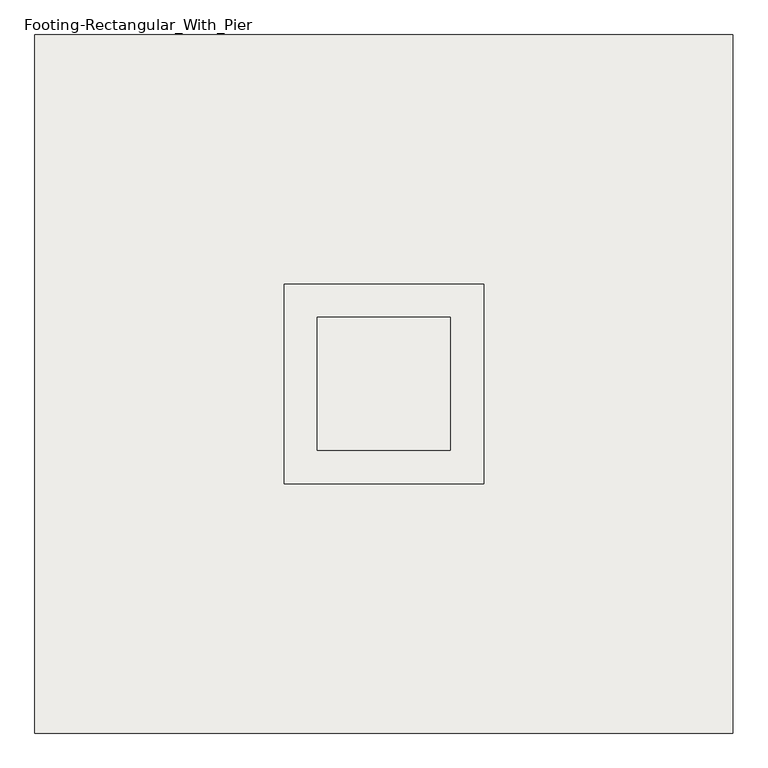
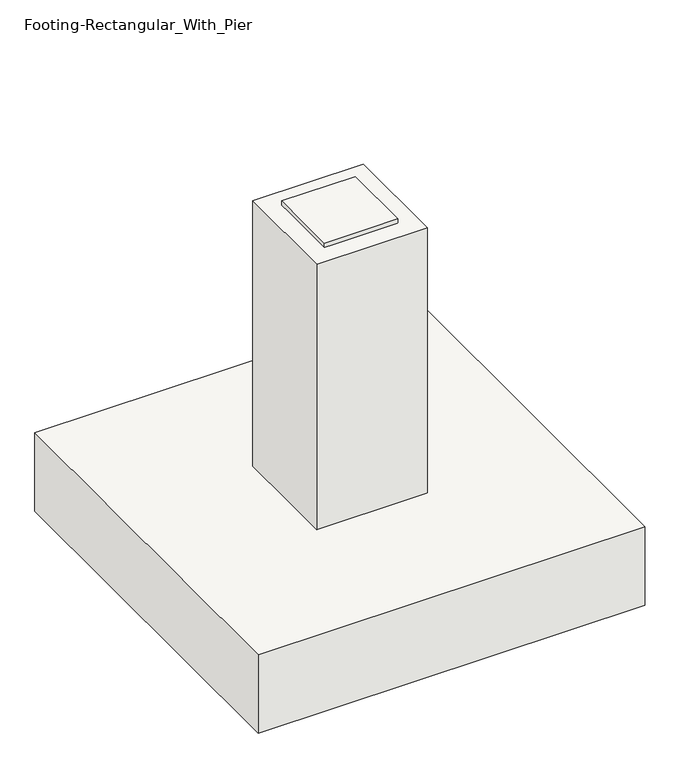
"""IFC4 building model written with IfcOpenShell, lengths in millimetres: slab geometry, Footing-Rectangular_With_Pier."""

import ifcopenshell
import ifcopenshell.guid

model = None  # the IFC model being written
_history = None  # IfcOwnerHistory: only IFC2X3 demands one
_inside = {}  # id of a spatial element -> (the spatial element, [elements in it])
_under = {}  # id of a project, library or spatial element -> (it, [spatial elements below it])
_declared = {}  # id of a project -> (the project, [libraries it declares])
_typed = {}  # id of a type object -> (the type object, [elements of that type])
_made_of = {}  # id of a material, layer set ... -> (it, [elements and type objects made of it])


def new_model(schema):
    """Start an empty IFC model of exactly this schema.

    Asked for "IFC4X3", IfcOpenShell would pick the latest addendum, in which some entities
    have other attributes; the version numbers below select the first issue.
    IFC2X3 requires an IfcOwnerHistory on every rooted entity: one is made here for all.
    """
    global model, _history
    if schema == "IFC4X3":
        model = ifcopenshell.file(schema_version=(4, 3, 0, 0))
    else:
        model = ifcopenshell.file(schema=schema)
    _inside.clear()
    _under.clear()
    _declared.clear()
    _typed.clear()
    _made_of.clear()
    _history = None
    if model.schema == "IFC2X3":
        org = make("IfcOrganization", Name="unknown")
        user = make(
            "IfcPersonAndOrganization",
            ThePerson=make("IfcPerson", FamilyName="unknown"),
            TheOrganization=org,
        )
        app = make(
            "IfcApplication",
            ApplicationDeveloper=org,
            Version="unknown",
            ApplicationFullName="unknown",
            ApplicationIdentifier="unknown",
        )
        _history = make(
            "IfcOwnerHistory",
            OwningUser=user,
            OwningApplication=app,
            ChangeAction="ADDED",
            CreationDate=0,
        )
    return model


def make(cls, **values):
    """One entity of the class cls with the attributes given. An attribute that is None is left unset."""
    return model.create_entity(
        cls, **{name: value for name, value in values.items() if value is not None}
    )


def rooted(cls, **values):
    """An entity with a GlobalId (a new one), such as an element, a storey or a relation."""
    return make(cls, GlobalId=ifcopenshell.guid.new(), OwnerHistory=_history, **values)


def si_unit(unit_type, name, prefix=None):
    """IfcSIUnit, for example si_unit("LENGTHUNIT", "METRE", prefix="MILLI")."""
    return make("IfcSIUnit", UnitType=unit_type, Prefix=prefix, Name=name)


def assignment(units):
    """IfcUnitAssignment: the units of a project."""
    return None if units is None else make("IfcUnitAssignment", Units=units)


def point(xyz):
    """IfcCartesianPoint."""
    return None if xyz is None else make("IfcCartesianPoint", Coordinates=xyz)


def direction(xyz):
    """IfcDirection."""
    return None if xyz is None else make("IfcDirection", DirectionRatios=xyz)


def frame(location, z_axis=None, x_axis=None):
    """IfcAxis2Placement3D, a coordinate frame: its origin and axes. An axis left out is left unset."""
    return make(
        "IfcAxis2Placement3D",
        Location=point(location),
        Axis=direction(z_axis),
        RefDirection=direction(x_axis),
    )


def origin():
    """The frame at (0, 0, 0) with its axes left unset."""
    return frame((0.0, 0.0, 0.0))


def origin_with_axes():
    """The frame at (0, 0, 0) with the z axis (0, 0, 1) and the x axis (1, 0, 0) written out."""
    return frame((0.0, 0.0, 0.0), z_axis=(0.0, 0.0, 1.0), x_axis=(1.0, 0.0, 0.0))


def place(relative_to, where):
    """IfcLocalPlacement: puts the frame where relative to a parent placement (None: the world)."""
    return make(
        "IfcLocalPlacement", PlacementRelTo=relative_to, RelativePlacement=where
    )


def context(
    kind, dimensions, precision=None, world=None, true_north=None, identifier=None
):
    """IfcGeometricRepresentationContext, for example the 3D "Model" context."""
    return make(
        "IfcGeometricRepresentationContext",
        ContextIdentifier=identifier,
        ContextType=kind,
        CoordinateSpaceDimension=dimensions,
        Precision=precision,
        WorldCoordinateSystem=world,
        TrueNorth=true_north,
    )


def project(units=None, contexts=None):
    """IfcProject with its units and contexts."""
    return rooted(
        "IfcProject",
        Name="project",
        RepresentationContexts=contexts,
        UnitsInContext=assignment(units),
    )


def spatial(cls, under=None, at=None, **own):
    """A site, building, storey or space (cls), placed at a placement, below another one or the project."""
    s = rooted(cls, ObjectPlacement=at, **own)
    if under is not None:
        _under.setdefault(under.id(), (under, []))[1].append(s)
    return s


def polyline(points):
    """IfcPolyline through the points."""
    return make("IfcPolyline", Points=[point(p) for p in points])


def outline(outer, holes=None, kind="AREA"):
    """IfcArbitraryClosedProfileDef: a profile drawn as a closed curve; with holes, ...WithVoids."""
    if holes is None:
        return make("IfcArbitraryClosedProfileDef", ProfileType=kind, OuterCurve=outer)
    return make(
        "IfcArbitraryProfileDefWithVoids",
        ProfileType=kind,
        OuterCurve=outer,
        InnerCurves=holes,
    )


def extrude(swept, where, along, depth):
    """IfcExtrudedAreaSolid: the profile swept, set in the frame where, extruded along a direction by depth."""
    return make(
        "IfcExtrudedAreaSolid",
        SweptArea=swept,
        Position=where,
        ExtrudedDirection=direction(along),
        Depth=depth,
    )


def shape(context_of_items, identifier, shape_type, items):
    """IfcShapeRepresentation: the items that make up one representation, for example the "Body"."""
    return make(
        "IfcShapeRepresentation",
        ContextOfItems=context_of_items,
        RepresentationIdentifier=identifier,
        RepresentationType=shape_type,
        Items=items,
    )


def source(mapping_origin, context_of_items, identifier, shape_type, items):
    """IfcRepresentationMap: a shape defined once, which mapped items show again and again."""
    return make(
        "IfcRepresentationMap",
        MappingOrigin=mapping_origin,
        MappedRepresentation=shape(context_of_items, identifier, shape_type, items),
    )


def transform(
    local_origin,
    x_axis=None,
    y_axis=None,
    z_axis=None,
    scale=None,
    scale2=None,
    scale3=None,
    uniform=True,
):
    """IfcCartesianTransformationOperator3D, or its non-uniform kind. x_axis, y_axis, z_axis: its Axis1, 2, 3."""
    if uniform:
        return make(
            "IfcCartesianTransformationOperator3D",
            Axis1=direction(x_axis),
            Axis2=direction(y_axis),
            LocalOrigin=point(local_origin),
            Scale=scale,
            Axis3=direction(z_axis),
        )
    return make(
        "IfcCartesianTransformationOperator3DnonUniform",
        Axis1=direction(x_axis),
        Axis2=direction(y_axis),
        LocalOrigin=point(local_origin),
        Scale=scale,
        Axis3=direction(z_axis),
        Scale2=scale2,
        Scale3=scale3,
    )


def mapped(mapping_source, mapping_target):
    """IfcMappedItem: shows the shape of a source again, moved by a transform."""
    return make(
        "IfcMappedItem", MappingSource=mapping_source, MappingTarget=mapping_target
    )


def made_of(thing, what):
    """Note that an element or type object is made of a material, layer set ...; save() writes the relation."""
    if what is not None:
        _made_of.setdefault(what.id(), (what, []))[1].append(thing)
    return thing


def element(
    cls,
    number,
    at=None,
    inside=None,
    cuts=None,
    type_object=None,
    material=None,
    context=None,
    identifier="Body",
    shape_type=None,
    held_by="IfcProductDefinitionShape",
    body=None,
    shapes=None,
    **own,
):
    """One element of the class cls, such as IfcWall. Its Tag is "e" and its number.

    at: its placement. inside: the storey or other place that contains it. cuts: it is an
    opening in that element (IfcRelVoidsElement). A single representation is given by context,
    identifier, shape_type and body (its items); several are given by shapes. held_by: the class
    of the entity that holds the representations. save() writes the other relations.
    """
    e = rooted(cls, Tag="e%d" % number, ObjectPlacement=at, **own)
    if body is not None:
        shapes = [shape(context, identifier, shape_type, body)]
    if shapes is not None:
        e.Representation = make(held_by, Representations=shapes)
    if inside is not None:
        _inside.setdefault(inside.id(), (inside, []))[1].append(e)
    if cuts is not None:
        rooted(
            "IfcRelVoidsElement", RelatingBuildingElement=cuts, RelatedOpeningElement=e
        )
    if type_object is not None:
        _typed.setdefault(type_object.id(), (type_object, []))[1].append(e)
    return made_of(e, material)


def aggregate(whole, parts):
    """IfcRelAggregates: a whole, such as a stair, and the parts it consists of."""
    return rooted("IfcRelAggregates", RelatingObject=whole, RelatedObjects=parts)


def save(model, path):
    """Write the relations noted so far, then the file.

    IfcRelAggregates (storeys below a building ...), IfcRelContainedInSpatialStructure (elements
    in a storey), IfcRelDefinesByType, IfcRelAssociatesMaterial and IfcRelDeclares: one each for
    every whole, place, type object, material and project.
    """
    for whole, parts in _under.values():
        aggregate(whole, parts)
    for where, things in _inside.values():
        rooted(
            "IfcRelContainedInSpatialStructure",
            RelatedElements=things,
            RelatingStructure=where,
        )
    for kind, things in _typed.values():
        rooted("IfcRelDefinesByType", RelatedObjects=things, RelatingType=kind)
    for what, things in _made_of.values():
        rooted("IfcRelAssociatesMaterial", RelatedObjects=things, RelatingMaterial=what)
    for by, libraries in _declared.values():
        rooted("IfcRelDeclares", RelatingContext=by, RelatedDefinitions=libraries)
    model.write(path)


def footing_rectangular_with_pier_64681127(model_context):
    return source(origin(), model_context, "Body", "SweptSolid", [
        extrude(outline(polyline([(203.2, 203.2), (203.2, -203.2), (-203.2, -203.2), (-203.2, 203.2), (203.2, 203.2)])), frame((0.0, 0.0, 1549.4), z_axis=(0.0, 0.0, 1.0), x_axis=(1.0, 0.0, 0.0)), (0.0, 0.0, 1.0), 25.4),
        extrude(outline(polyline([(1066.8, 1066.8), (1066.8, -1066.8), (-1066.8, -1066.8), (-1066.8, 1066.8), (1066.8, 1066.8)])), frame((0.0, 0.0, -457.2), z_axis=(0.0, 0.0, 1.0), x_axis=(1.0, 0.0, 0.0)), (0.0, 0.0, 1.0), 457.2),
        extrude(outline(polyline([(304.8, 304.8), (304.8, -304.8), (-304.8, -304.8), (-304.8, 304.8), (304.8, 304.8)])), origin_with_axes(), (0.0, 0.0, 1.0), 1549.4),
    ])


if __name__ == "__main__":
    model = new_model("IFC4")
    model_context = context("Model", 3, world=origin())
    ifc_project = project(units=[si_unit("LENGTHUNIT", "METRE", prefix="MILLI")], contexts=[model_context])
    site = spatial("IfcSite", under=ifc_project)
    building = spatial("IfcBuilding", under=site)
    placement = place(None, origin())
    footing_rectangular_with_pier_shape = footing_rectangular_with_pier_64681127(model_context)
    element("IfcSlab", 1, ObjectType="Footing-Rectangular_With_Pier : F6 - 7'-0\" x 7'-0\" x 1'-6\"", at=placement, inside=building, context=model_context, shape_type="MappedRepresentation", body=[
        mapped(footing_rectangular_with_pier_shape, transform((0.0, 0.0, 0.0), x_axis=(1.0, 0.0, 0.0), y_axis=(0.0, 1.0, 0.0), z_axis=(0.0, 0.0, 1.0))),
    ])
    save(model, "model.ifc")

# Revit data of these elements
# Type "Footing-Rectangular_With_Pier : F6 - 7'-0\" x 7'-0\" x 1'-6\""
#   Type Mark = "F6"
#   Assembly Code = "A1010100"
#   Width = 2133.6 mm
#   SteelPlateWidth [instance default] = 406.4 mm
#   SteelPlateThickness [instance default] = 25.4 mm
#   SteelPlateDepth [instance default] = 406.4 mm
#   PierWidth [instance default] = 609.6 mm
#   PierLength [instance default] = 609.6 mm
#   PierDepth [instance default] = 1371.6 mm
#   Length = 2133.6 mm
#   FootingThickness = 457.2 mm
#   Steel Plate = yes
#   Structural Material [instance default] = Concrete - Cast-in-Place Concrete
# Element 1 (IfcSlab, "Footing-Rectangular_With_Pier : F6 - 7'-0\" x 7'-0\" x 1'-6\"")
#   PierDepth = 1549.4 mm
#   Materials on its faces: "Concrete - Cast-in-Place Concrete", "Steel"
# Materials
#   "Concrete - Cast-in-Place Concrete": class "Concrete", colour RGB 192 192 192, transparency 0
#   "Steel": class "Metal", colour RGB 247 247 247, transparency 0, Description = "Steel, mill finish", Cost = 0
